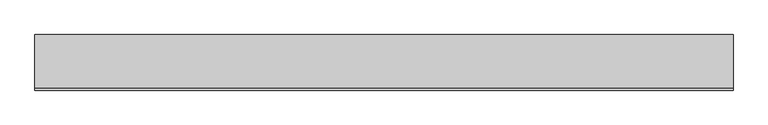
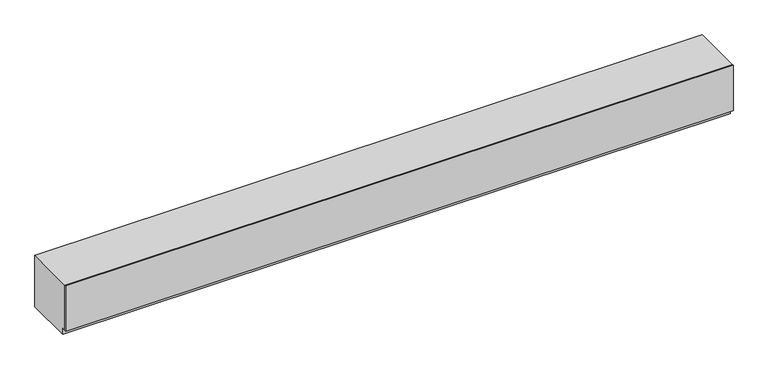
"""IFC4 building model written with IfcOpenShell, lengths in millimetres: furniture geometry, OD_CW_Base Cabinet : OD_CW_Base Cabinet."""

import ifcopenshell
import ifcopenshell.guid

model = None  # the IFC model being written
_history = None  # IfcOwnerHistory: only IFC2X3 demands one
_inside = {}  # id of a spatial element -> (the spatial element, [elements in it])
_under = {}  # id of a project, library or spatial element -> (it, [spatial elements below it])
_declared = {}  # id of a project -> (the project, [libraries it declares])
_typed = {}  # id of a type object -> (the type object, [elements of that type])
_made_of = {}  # id of a material, layer set ... -> (it, [elements and type objects made of it])


def new_model(schema):
    """Start an empty IFC model of exactly this schema.

    Asked for "IFC4X3", IfcOpenShell would pick the latest addendum, in which some entities
    have other attributes; the version numbers below select the first issue.
    IFC2X3 requires an IfcOwnerHistory on every rooted entity: one is made here for all.
    """
    global model, _history
    if schema == "IFC4X3":
        model = ifcopenshell.file(schema_version=(4, 3, 0, 0))
    else:
        model = ifcopenshell.file(schema=schema)
    _inside.clear()
    _under.clear()
    _declared.clear()
    _typed.clear()
    _made_of.clear()
    _history = None
    if model.schema == "IFC2X3":
        org = make("IfcOrganization", Name="unknown")
        user = make(
            "IfcPersonAndOrganization",
            ThePerson=make("IfcPerson", FamilyName="unknown"),
            TheOrganization=org,
        )
        app = make(
            "IfcApplication",
            ApplicationDeveloper=org,
            Version="unknown",
            ApplicationFullName="unknown",
            ApplicationIdentifier="unknown",
        )
        _history = make(
            "IfcOwnerHistory",
            OwningUser=user,
            OwningApplication=app,
            ChangeAction="ADDED",
            CreationDate=0,
        )
    return model


def make(cls, **values):
    """One entity of the class cls with the attributes given. An attribute that is None is left unset."""
    return model.create_entity(
        cls, **{name: value for name, value in values.items() if value is not None}
    )


def rooted(cls, **values):
    """An entity with a GlobalId (a new one), such as an element, a storey or a relation."""
    return make(cls, GlobalId=ifcopenshell.guid.new(), OwnerHistory=_history, **values)


def si_unit(unit_type, name, prefix=None):
    """IfcSIUnit, for example si_unit("LENGTHUNIT", "METRE", prefix="MILLI")."""
    return make("IfcSIUnit", UnitType=unit_type, Prefix=prefix, Name=name)


def assignment(units):
    """IfcUnitAssignment: the units of a project."""
    return None if units is None else make("IfcUnitAssignment", Units=units)


def point(xyz):
    """IfcCartesianPoint."""
    return None if xyz is None else make("IfcCartesianPoint", Coordinates=xyz)


def direction(xyz):
    """IfcDirection."""
    return None if xyz is None else make("IfcDirection", DirectionRatios=xyz)


def frame(location, z_axis=None, x_axis=None):
    """IfcAxis2Placement3D, a coordinate frame: its origin and axes. An axis left out is left unset."""
    return make(
        "IfcAxis2Placement3D",
        Location=point(location),
        Axis=direction(z_axis),
        RefDirection=direction(x_axis),
    )


def origin():
    """The frame at (0, 0, 0) with its axes left unset."""
    return frame((0.0, 0.0, 0.0))


def place(relative_to, where):
    """IfcLocalPlacement: puts the frame where relative to a parent placement (None: the world)."""
    return make(
        "IfcLocalPlacement", PlacementRelTo=relative_to, RelativePlacement=where
    )


def context(
    kind, dimensions, precision=None, world=None, true_north=None, identifier=None
):
    """IfcGeometricRepresentationContext, for example the 3D "Model" context."""
    return make(
        "IfcGeometricRepresentationContext",
        ContextIdentifier=identifier,
        ContextType=kind,
        CoordinateSpaceDimension=dimensions,
        Precision=precision,
        WorldCoordinateSystem=world,
        TrueNorth=true_north,
    )


def project(units=None, contexts=None):
    """IfcProject with its units and contexts."""
    return rooted(
        "IfcProject",
        Name="project",
        RepresentationContexts=contexts,
        UnitsInContext=assignment(units),
    )


def spatial(cls, under=None, at=None, **own):
    """A site, building, storey or space (cls), placed at a placement, below another one or the project."""
    s = rooted(cls, ObjectPlacement=at, **own)
    if under is not None:
        _under.setdefault(under.id(), (under, []))[1].append(s)
    return s


def polyline(points):
    """IfcPolyline through the points."""
    return make("IfcPolyline", Points=[point(p) for p in points])


def outline(outer, holes=None, kind="AREA"):
    """IfcArbitraryClosedProfileDef: a profile drawn as a closed curve; with holes, ...WithVoids."""
    if holes is None:
        return make("IfcArbitraryClosedProfileDef", ProfileType=kind, OuterCurve=outer)
    return make(
        "IfcArbitraryProfileDefWithVoids",
        ProfileType=kind,
        OuterCurve=outer,
        InnerCurves=holes,
    )


def extrude(swept, where, along, depth):
    """IfcExtrudedAreaSolid: the profile swept, set in the frame where, extruded along a direction by depth."""
    return make(
        "IfcExtrudedAreaSolid",
        SweptArea=swept,
        Position=where,
        ExtrudedDirection=direction(along),
        Depth=depth,
    )


def shape(context_of_items, identifier, shape_type, items):
    """IfcShapeRepresentation: the items that make up one representation, for example the "Body"."""
    return make(
        "IfcShapeRepresentation",
        ContextOfItems=context_of_items,
        RepresentationIdentifier=identifier,
        RepresentationType=shape_type,
        Items=items,
    )


def source(mapping_origin, context_of_items, identifier, shape_type, items):
    """IfcRepresentationMap: a shape defined once, which mapped items show again and again."""
    return make(
        "IfcRepresentationMap",
        MappingOrigin=mapping_origin,
        MappedRepresentation=shape(context_of_items, identifier, shape_type, items),
    )


def transform(
    local_origin,
    x_axis=None,
    y_axis=None,
    z_axis=None,
    scale=None,
    scale2=None,
    scale3=None,
    uniform=True,
):
    """IfcCartesianTransformationOperator3D, or its non-uniform kind. x_axis, y_axis, z_axis: its Axis1, 2, 3."""
    if uniform:
        return make(
            "IfcCartesianTransformationOperator3D",
            Axis1=direction(x_axis),
            Axis2=direction(y_axis),
            LocalOrigin=point(local_origin),
            Scale=scale,
            Axis3=direction(z_axis),
        )
    return make(
        "IfcCartesianTransformationOperator3DnonUniform",
        Axis1=direction(x_axis),
        Axis2=direction(y_axis),
        LocalOrigin=point(local_origin),
        Scale=scale,
        Axis3=direction(z_axis),
        Scale2=scale2,
        Scale3=scale3,
    )


def mapped(mapping_source, mapping_target):
    """IfcMappedItem: shows the shape of a source again, moved by a transform."""
    return make(
        "IfcMappedItem", MappingSource=mapping_source, MappingTarget=mapping_target
    )


def made_of(thing, what):
    """Note that an element or type object is made of a material, layer set ...; save() writes the relation."""
    if what is not None:
        _made_of.setdefault(what.id(), (what, []))[1].append(thing)
    return thing


def element(
    cls,
    number,
    at=None,
    inside=None,
    cuts=None,
    type_object=None,
    material=None,
    context=None,
    identifier="Body",
    shape_type=None,
    held_by="IfcProductDefinitionShape",
    body=None,
    shapes=None,
    **own,
):
    """One element of the class cls, such as IfcWall. Its Tag is "e" and its number.

    at: its placement. inside: the storey or other place that contains it. cuts: it is an
    opening in that element (IfcRelVoidsElement). A single representation is given by context,
    identifier, shape_type and body (its items); several are given by shapes. held_by: the class
    of the entity that holds the representations. save() writes the other relations.
    """
    e = rooted(cls, Tag="e%d" % number, ObjectPlacement=at, **own)
    if body is not None:
        shapes = [shape(context, identifier, shape_type, body)]
    if shapes is not None:
        e.Representation = make(held_by, Representations=shapes)
    if inside is not None:
        _inside.setdefault(inside.id(), (inside, []))[1].append(e)
    if cuts is not None:
        rooted(
            "IfcRelVoidsElement", RelatingBuildingElement=cuts, RelatedOpeningElement=e
        )
    if type_object is not None:
        _typed.setdefault(type_object.id(), (type_object, []))[1].append(e)
    return made_of(e, material)


def aggregate(whole, parts):
    """IfcRelAggregates: a whole, such as a stair, and the parts it consists of."""
    return rooted("IfcRelAggregates", RelatingObject=whole, RelatedObjects=parts)


def save(model, path):
    """Write the relations noted so far, then the file.

    IfcRelAggregates (storeys below a building ...), IfcRelContainedInSpatialStructure (elements
    in a storey), IfcRelDefinesByType, IfcRelAssociatesMaterial and IfcRelDeclares: one each for
    every whole, place, type object, material and project.
    """
    for whole, parts in _under.values():
        aggregate(whole, parts)
    for where, things in _inside.values():
        rooted(
            "IfcRelContainedInSpatialStructure",
            RelatedElements=things,
            RelatingStructure=where,
        )
    for kind, things in _typed.values():
        rooted("IfcRelDefinesByType", RelatedObjects=things, RelatingType=kind)
    for what, things in _made_of.values():
        rooted("IfcRelAssociatesMaterial", RelatedObjects=things, RelatingMaterial=what)
    for by, libraries in _declared.values():
        rooted("IfcRelDeclares", RelatingContext=by, RelatedDefinitions=libraries)
    model.write(path)


def furniture_29fa6a70(model_context):
    return source(origin(), model_context, "Body", "SweptSolid", [
        extrude(outline(polyline([(18.7377049, -228.6), (10849.5020576, -228.6), (10849.5020576, -254.0), (18.7377049, -254.0), (18.7377049, -228.6)])), frame((0.0, 0.0, 101.6), z_axis=(0.0, 0.0, 1.0), x_axis=(1.0, 0.0, 0.0)), (0.0, 0.0, 1.0), 774.7),
        extrude(outline(polyline([(-228.6, 876.3), (609.6, 876.3), (609.6, 0.0), (-177.8, 0.0), (-177.8, 101.6), (-228.6, 101.6), (-228.6, 876.3)])), frame((18.7377049, 0.0, 0.0), z_axis=(1.0, 0.0, 0.0), x_axis=(0.0, 1.0, 0.0)), (0.0, 0.0, 1.0), 10830.7643527),
    ])


if __name__ == "__main__":
    model = new_model("IFC4")
    model_context = context("Model", 3, world=origin())
    ifc_project = project(units=[si_unit("LENGTHUNIT", "METRE", prefix="MILLI")], contexts=[model_context])
    site = spatial("IfcSite", under=ifc_project)
    building = spatial("IfcBuilding", under=site)
    placement = place(None, origin())
    furniture_shape = furniture_29fa6a70(model_context)
    element("IfcFurniture", 1, ObjectType="OD_CW_Base Cabinet : OD_CW_Base Cabinet", at=placement, inside=building, context=model_context, shape_type="MappedRepresentation", body=[
        mapped(furniture_shape, transform((0.0, 0.0, 0.0), x_axis=(1.0, 0.0, 0.0), y_axis=(0.0, 1.0, 0.0), z_axis=(0.0, 0.0, 1.0))),
    ])
    save(model, "model.ifc")

# Revit data of these elements
# Type "OD_CW_Base Cabinet : OD_CW_Base Cabinet"
#   OD_CW_Width [instance default] = 2' - 10"
#   OD_CW_Length [instance default] = 8' - 0"
#   OD_CW_Height [instance default] = 2' - 3"
#   Depth = 2' - 0"
#   Height = 3' - 0"
#   Width = 4' - 0"
#   OD_CW_Material_Front Panel [instance default] = none
#   OD_CW_Material_Body [instance default] = none
# Element 1 (IfcFurniture, "OD_CW_Base Cabinet : OD_CW_Base Cabinet")
#   OD_CW_Length = 35' - 6.40805"
#   OD_CW_Height = 2' - 10 1/2"
#   Materials on its faces: "CASEWORK"
# Materials
#   "CASEWORK": class "Generic", colour RGB 181 181 181, transparency 0, Cost = 0
